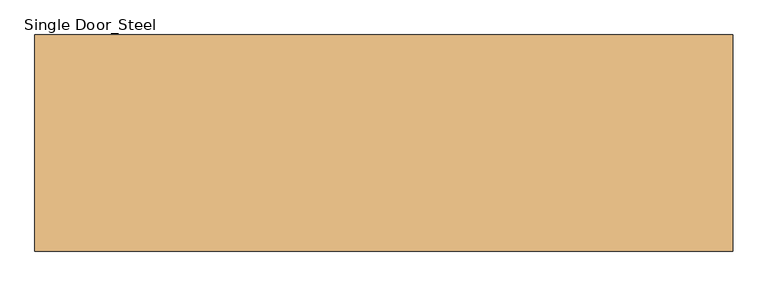
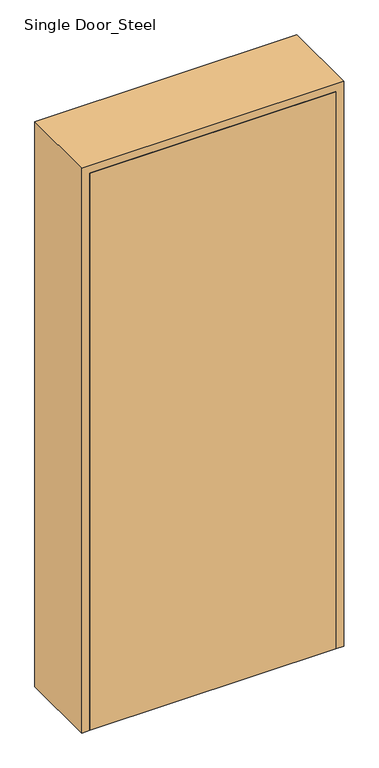
"""IFC4 building model written with IfcOpenShell, lengths in millimetres: door geometry, Single Door_Steel : H_DR_AR_B12_Single Door_Steel_W1000xH2280_FSD1."""

from ifc_helpers import new_model, si_unit, origin, origin_with_axes, place, context, project, spatial, polyline, outline, extrude, faceted_brep, source, transform, mapped, element, save


def single_door_steel_001f4ee4(model_context):
    return source(origin(), model_context, "Body", "SolidModel", [
        extrude(outline(polyline([(470.0, -155.0), (-470.0, -155.0), (-470.0, -120.0), (470.0, -120.0), (470.0, -155.0)])), origin_with_axes(), (0.0, 0.0, 1.0), 2250.0),
        faceted_brep([(470.0, -155.0, 0.0), (470.0, -120.0, 0.0), (450.0, -120.0, 0.0), (450.0, 120.0, 0.0), (470.0, 120.0, 0.0), (470.0, 155.0, 0.0), (500.0, 155.0, 0.0), (500.0, -155.0, 0.0), (500.0, -155.0, 2280.0), (-500.0, -155.0, 2280.0), (-500.0, -155.0, 0.0), (-470.0, -155.0, 0.0), (-470.0, -155.0, 2250.0), (470.0, -155.0, 2250.0), (500.0, 155.0, 2280.0), (470.0, 155.0, 2250.0), (-470.0, 155.0, 2250.0), (-470.0, 155.0, 0.0), (-500.0, 155.0, 0.0), (-500.0, 155.0, 2280.0), (470.0, 120.0, 2250.0), (450.0, 120.0, 2230.0), (-450.0, 120.0, 2230.0), (-450.0, 120.0, 0.0), (-470.0, 120.0, 0.0), (-470.0, 120.0, 2250.0), (450.0, -120.0, 2230.0), (470.0, -120.0, 2250.0), (-470.0, -120.0, 2250.0), (-470.0, -120.0, 0.0), (-450.0, -120.0, 0.0), (-450.0, -120.0, 2230.0)], [[[0, 1, 2, 3, 4, 5, 6, 7]], [[7, 8, 9, 10, 11, 12, 13, 0]], [[6, 14, 8, 7]], [[5, 15, 16, 17, 18, 19, 14, 6]], [[4, 20, 15, 5]], [[3, 21, 22, 23, 24, 25, 20, 4]], [[2, 26, 21, 3]], [[1, 27, 28, 29, 30, 31, 26, 2]], [[0, 13, 27, 1]], [[12, 11, 29, 28]], [[11, 10, 18, 17, 24, 23, 30, 29]], [[19, 18, 10, 9]], [[25, 24, 17, 16]], [[31, 30, 23, 22]], [[14, 19, 9, 8]], [[20, 25, 16, 15]], [[26, 31, 22, 21]], [[13, 12, 28, 27]]]),
    ])


if __name__ == "__main__":
    model = new_model("IFC4")
    model_context = context("Model", 3, world=origin())
    ifc_project = project(units=[si_unit("LENGTHUNIT", "METRE", prefix="MILLI")], contexts=[model_context])
    site = spatial("IfcSite", under=ifc_project)
    building = spatial("IfcBuilding", under=site)
    placement = place(None, origin())
    single_door_steel_shape = single_door_steel_001f4ee4(model_context)
    element("IfcDoor", 1, ObjectType="Single Door_Steel : H_DR_AR_B12_Single Door_Steel_W1000xH2280_FSD1", at=placement, inside=building, context=model_context, shape_type="MappedRepresentation", body=[
        mapped(single_door_steel_shape, transform((0.0, 0.0, 0.0), x_axis=(1.0, 0.0, 0.0), y_axis=(0.0, 1.0, 0.0), z_axis=(0.0, 0.0, 1.0))),
    ])
    save(model, "model.ifc")

# Revit data of these elements
# Type "Single Door_Steel : H_DR_AR_B12_Single Door_Steel_W1000xH2280_FSD1"
#   Type Mark = "439"
#   Analytic Construction = "<None>"
#   프레임 투영 외부. = 25 mm
#   프레임 투영 내부. = 25 mm
#   프레임 폭 = 75 mm
#   Height = 2280 mm
#   Width = 1000 mm
#   Define Thermal Properties by = 1
#   문 패널 = none
#   문 프레임 = none
#   Function = (empty or 0)
#   Wall Closure = (empty or 0)
